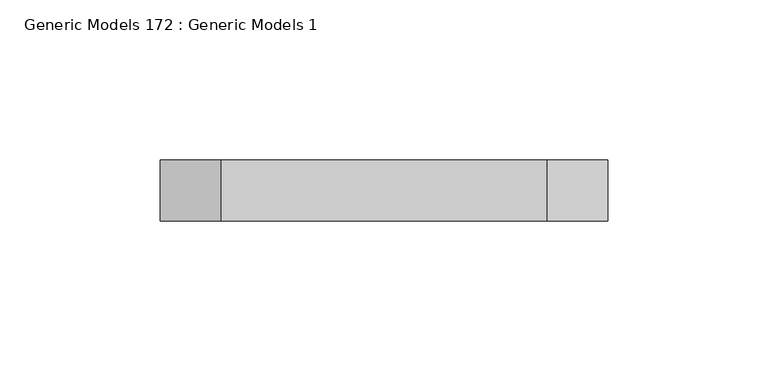
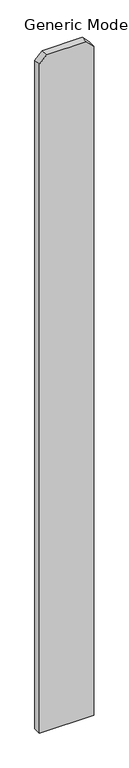
"""IFC4 building model written with IfcOpenShell, lengths in millimetres: proxy geometry, Generic Models 172 : Generic Models 1."""

from ifc_helpers import new_model, si_unit, frame, origin, place, context, project, spatial, polyline, outline, extrude, source, transform, mapped, element, save


def generic_models_172_generic_models_1_01be16c1(model_context):
    return source(origin(), model_context, "Body", "SweptSolid", [
        extrude(outline(polyline([(76.2, 56208.6125), (1885.95, 56208.6125), (1905.0, 56189.5625), (1905.0, 56087.9625), (1885.95, 56068.9125), (76.2, 56068.9125), (76.2, 56208.6125)])), frame((0.0, 547.6875, 0.0), z_axis=(0.0, 1.0, 0.0), x_axis=(0.0, 0.0, 1.0)), (0.0, 0.0, 1.0), 19.05),
    ])


if __name__ == "__main__":
    model = new_model("IFC4")
    model_context = context("Model", 3, world=origin())
    ifc_project = project(units=[si_unit("LENGTHUNIT", "METRE", prefix="MILLI")], contexts=[model_context])
    site = spatial("IfcSite", under=ifc_project)
    building = spatial("IfcBuilding", under=site)
    placement = place(None, origin())
    generic_models_172_generic_models_1_shape = generic_models_172_generic_models_1_01be16c1(model_context)
    element("IfcBuildingElementProxy", 1, Name="Generic Models 172 : Generic Models 1", ObjectType="Generic Models 172 : Generic Models 1", at=placement, inside=building, context=model_context, shape_type="MappedRepresentation", body=[
        mapped(generic_models_172_generic_models_1_shape, transform((0.0, 0.0, 0.0), x_axis=(1.0, 0.0, 0.0), y_axis=(0.0, 1.0, 0.0), z_axis=(0.0, 0.0, 1.0))),
    ])
    save(model, "model.ifc")

# Revit data of these elements
# Element 1 (IfcBuildingElementProxy, "Generic Models 172 : Generic Models 1")
#   Materials on its faces: "VERTICAL 1X6 CEDAR PLANKS W/ CLEAR WOOD SEALER"
# Materials
#   "VERTICAL 1X6 CEDAR PLANKS W/ CLEAR WOOD SEALER": class "Wood", colour RGB 234 198 147, transparency 0, Description = "Pinus Echinata", Cost = 0
